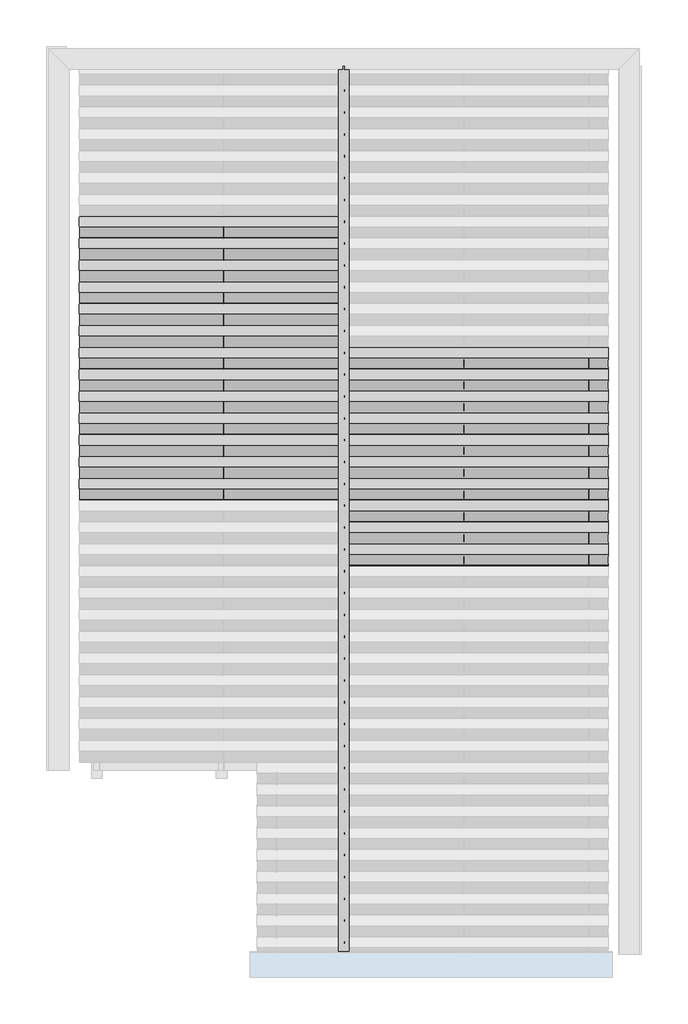
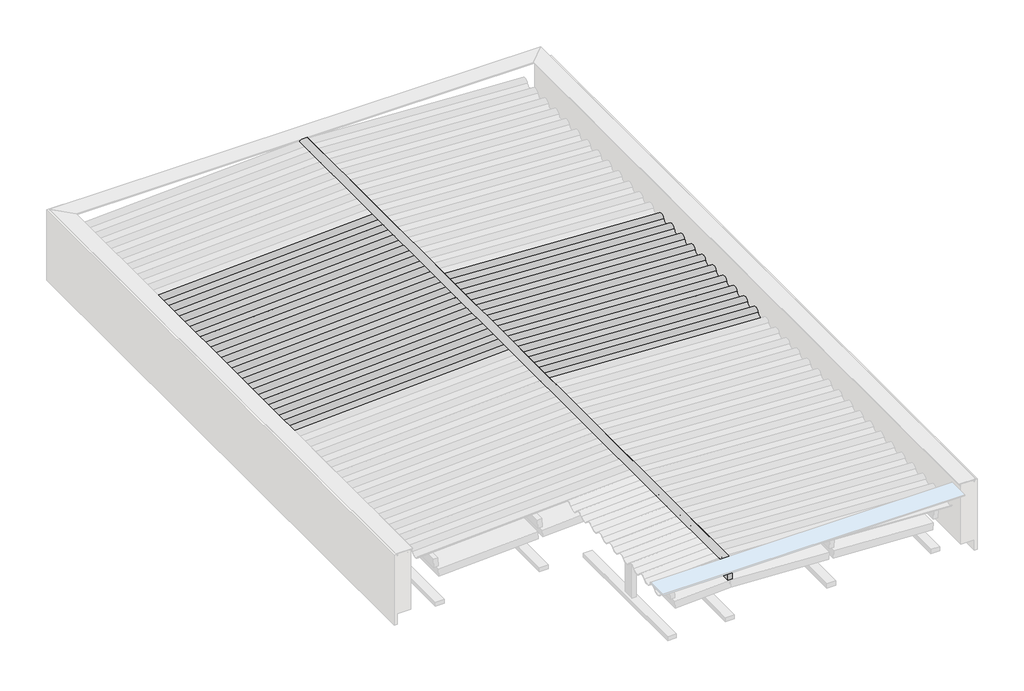
# One storey, part 3 of 4: 32 beams, 6 columns.
"""IFC4 building model written with IfcOpenShell, lengths in millimetres."""

import ifcopenshell
import ifcopenshell.guid

model = None  # the IFC model being written
_history = None  # IfcOwnerHistory: only IFC2X3 demands one
_inside = {}  # id of a spatial element -> (the spatial element, [elements in it])
_under = {}  # id of a project, library or spatial element -> (it, [spatial elements below it])
_declared = {}  # id of a project -> (the project, [libraries it declares])
_typed = {}  # id of a type object -> (the type object, [elements of that type])
_made_of = {}  # id of a material, layer set ... -> (it, [elements and type objects made of it])


def new_model(schema):
    """Start an empty IFC model of exactly this schema.

    Asked for "IFC4X3", IfcOpenShell would pick the latest addendum, in which some entities
    have other attributes; the version numbers below select the first issue.
    IFC2X3 requires an IfcOwnerHistory on every rooted entity: one is made here for all.
    """
    global model, _history
    if schema == "IFC4X3":
        model = ifcopenshell.file(schema_version=(4, 3, 0, 0))
    else:
        model = ifcopenshell.file(schema=schema)
    _inside.clear()
    _under.clear()
    _declared.clear()
    _typed.clear()
    _made_of.clear()
    _history = None
    if model.schema == "IFC2X3":
        org = make("IfcOrganization", Name="unknown")
        user = make(
            "IfcPersonAndOrganization",
            ThePerson=make("IfcPerson", FamilyName="unknown"),
            TheOrganization=org,
        )
        app = make(
            "IfcApplication",
            ApplicationDeveloper=org,
            Version="unknown",
            ApplicationFullName="unknown",
            ApplicationIdentifier="unknown",
        )
        _history = make(
            "IfcOwnerHistory",
            OwningUser=user,
            OwningApplication=app,
            ChangeAction="ADDED",
            CreationDate=0,
        )
    return model


def make(cls, **values):
    """One entity of the class cls with the attributes given. An attribute that is None is left unset."""
    return model.create_entity(
        cls, **{name: value for name, value in values.items() if value is not None}
    )


def rooted(cls, **values):
    """An entity with a GlobalId (a new one), such as an element, a storey or a relation."""
    return make(cls, GlobalId=ifcopenshell.guid.new(), OwnerHistory=_history, **values)


def si_unit(unit_type, name, prefix=None):
    """IfcSIUnit, for example si_unit("LENGTHUNIT", "METRE", prefix="MILLI")."""
    return make("IfcSIUnit", UnitType=unit_type, Prefix=prefix, Name=name)


def assignment(units):
    """IfcUnitAssignment: the units of a project."""
    return None if units is None else make("IfcUnitAssignment", Units=units)


def point(xyz):
    """IfcCartesianPoint."""
    return None if xyz is None else make("IfcCartesianPoint", Coordinates=xyz)


def direction(xyz):
    """IfcDirection."""
    return None if xyz is None else make("IfcDirection", DirectionRatios=xyz)


def frame(location, z_axis=None, x_axis=None):
    """IfcAxis2Placement3D, a coordinate frame: its origin and axes. An axis left out is left unset."""
    return make(
        "IfcAxis2Placement3D",
        Location=point(location),
        Axis=direction(z_axis),
        RefDirection=direction(x_axis),
    )


def frame_2d(location, x_axis=None):
    """IfcAxis2Placement2D, a coordinate frame in the plane: its origin and x axis."""
    return make(
        "IfcAxis2Placement2D", Location=point(location), RefDirection=direction(x_axis)
    )


def origin():
    """The frame at (0, 0, 0) with its axes left unset."""
    return frame((0.0, 0.0, 0.0))


def place(relative_to, where):
    """IfcLocalPlacement: puts the frame where relative to a parent placement (None: the world)."""
    return make(
        "IfcLocalPlacement", PlacementRelTo=relative_to, RelativePlacement=where
    )


def context(
    kind, dimensions, precision=None, world=None, true_north=None, identifier=None
):
    """IfcGeometricRepresentationContext, for example the 3D "Model" context."""
    return make(
        "IfcGeometricRepresentationContext",
        ContextIdentifier=identifier,
        ContextType=kind,
        CoordinateSpaceDimension=dimensions,
        Precision=precision,
        WorldCoordinateSystem=world,
        TrueNorth=true_north,
    )


def project(units=None, contexts=None):
    """IfcProject with its units and contexts."""
    return rooted(
        "IfcProject",
        Name="project",
        RepresentationContexts=contexts,
        UnitsInContext=assignment(units),
    )


def spatial(cls, under=None, at=None, **own):
    """A site, building, storey or space (cls), placed at a placement, below another one or the project."""
    s = rooted(cls, ObjectPlacement=at, **own)
    if under is not None:
        _under.setdefault(under.id(), (under, []))[1].append(s)
    return s


def polyline(points):
    """IfcPolyline through the points."""
    return make("IfcPolyline", Points=[point(p) for p in points])


def circle_curve(where, radius):
    """IfcCircle in the frame where."""
    return make("IfcCircle", Position=where, Radius=radius)


def trimmed(basis, trim1, trim2, sense, master):
    """IfcTrimmedCurve: the piece of a basis curve between two trims."""
    return make(
        "IfcTrimmedCurve",
        BasisCurve=basis,
        Trim1=trim1,
        Trim2=trim2,
        SenseAgreement=sense,
        MasterRepresentation=master,
    )


def segment(curve, same_sense, transition):
    """IfcCompositeCurveSegment."""
    return make(
        "IfcCompositeCurveSegment",
        Transition=transition,
        SameSense=same_sense,
        ParentCurve=curve,
    )


def composite_curve(segments, self_intersect=None):
    """IfcCompositeCurve: segments joined end to end."""
    return make("IfcCompositeCurve", Segments=segments, SelfIntersect=self_intersect)


def outline(outer, holes=None, kind="AREA"):
    """IfcArbitraryClosedProfileDef: a profile drawn as a closed curve; with holes, ...WithVoids."""
    if holes is None:
        return make("IfcArbitraryClosedProfileDef", ProfileType=kind, OuterCurve=outer)
    return make(
        "IfcArbitraryProfileDefWithVoids",
        ProfileType=kind,
        OuterCurve=outer,
        InnerCurves=holes,
    )


def extrude(swept, where, along, depth):
    """IfcExtrudedAreaSolid: the profile swept, set in the frame where, extruded along a direction by depth."""
    return make(
        "IfcExtrudedAreaSolid",
        SweptArea=swept,
        Position=where,
        ExtrudedDirection=direction(along),
        Depth=depth,
    )


def shape(context_of_items, identifier, shape_type, items):
    """IfcShapeRepresentation: the items that make up one representation, for example the "Body"."""
    return make(
        "IfcShapeRepresentation",
        ContextOfItems=context_of_items,
        RepresentationIdentifier=identifier,
        RepresentationType=shape_type,
        Items=items,
    )


def source(mapping_origin, context_of_items, identifier, shape_type, items):
    """IfcRepresentationMap: a shape defined once, which mapped items show again and again."""
    return make(
        "IfcRepresentationMap",
        MappingOrigin=mapping_origin,
        MappedRepresentation=shape(context_of_items, identifier, shape_type, items),
    )


def transform(
    local_origin,
    x_axis=None,
    y_axis=None,
    z_axis=None,
    scale=None,
    scale2=None,
    scale3=None,
    uniform=True,
):
    """IfcCartesianTransformationOperator3D, or its non-uniform kind. x_axis, y_axis, z_axis: its Axis1, 2, 3."""
    if uniform:
        return make(
            "IfcCartesianTransformationOperator3D",
            Axis1=direction(x_axis),
            Axis2=direction(y_axis),
            LocalOrigin=point(local_origin),
            Scale=scale,
            Axis3=direction(z_axis),
        )
    return make(
        "IfcCartesianTransformationOperator3DnonUniform",
        Axis1=direction(x_axis),
        Axis2=direction(y_axis),
        LocalOrigin=point(local_origin),
        Scale=scale,
        Axis3=direction(z_axis),
        Scale2=scale2,
        Scale3=scale3,
    )


def mapped(mapping_source, mapping_target):
    """IfcMappedItem: shows the shape of a source again, moved by a transform."""
    return make(
        "IfcMappedItem", MappingSource=mapping_source, MappingTarget=mapping_target
    )


def made_of(thing, what):
    """Note that an element or type object is made of a material, layer set ...; save() writes the relation."""
    if what is not None:
        _made_of.setdefault(what.id(), (what, []))[1].append(thing)
    return thing


def element(
    cls,
    number,
    at=None,
    inside=None,
    cuts=None,
    type_object=None,
    material=None,
    context=None,
    identifier="Body",
    shape_type=None,
    held_by="IfcProductDefinitionShape",
    body=None,
    shapes=None,
    **own,
):
    """One element of the class cls, such as IfcWall. Its Tag is "e" and its number.

    at: its placement. inside: the storey or other place that contains it. cuts: it is an
    opening in that element (IfcRelVoidsElement). A single representation is given by context,
    identifier, shape_type and body (its items); several are given by shapes. held_by: the class
    of the entity that holds the representations. save() writes the other relations.
    """
    e = rooted(cls, Tag="e%d" % number, ObjectPlacement=at, **own)
    if body is not None:
        shapes = [shape(context, identifier, shape_type, body)]
    if shapes is not None:
        e.Representation = make(held_by, Representations=shapes)
    if inside is not None:
        _inside.setdefault(inside.id(), (inside, []))[1].append(e)
    if cuts is not None:
        rooted(
            "IfcRelVoidsElement", RelatingBuildingElement=cuts, RelatedOpeningElement=e
        )
    if type_object is not None:
        _typed.setdefault(type_object.id(), (type_object, []))[1].append(e)
    return made_of(e, material)


def aggregate(whole, parts):
    """IfcRelAggregates: a whole, such as a stair, and the parts it consists of."""
    return rooted("IfcRelAggregates", RelatingObject=whole, RelatedObjects=parts)


def save(model, path):
    """Write the relations noted so far, then the file.

    IfcRelAggregates (storeys below a building ...), IfcRelContainedInSpatialStructure (elements
    in a storey), IfcRelDefinesByType, IfcRelAssociatesMaterial and IfcRelDeclares: one each for
    every whole, place, type object, material and project.
    """
    for whole, parts in _under.values():
        aggregate(whole, parts)
    for where, things in _inside.values():
        rooted(
            "IfcRelContainedInSpatialStructure",
            RelatedElements=things,
            RelatingStructure=where,
        )
    for kind, things in _typed.values():
        rooted("IfcRelDefinesByType", RelatedObjects=things, RelatingType=kind)
    for what, things in _made_of.values():
        rooted("IfcRelAssociatesMaterial", RelatedObjects=things, RelatingMaterial=what)
    for by, libraries in _declared.values():
        rooted("IfcRelDeclares", RelatingContext=by, RelatedDefinitions=libraries)
    model.write(path)


def cumeeira_telha_ondulada_fibrocimento_c9eafb3e(model_context):
    return source(origin(), model_context, "Body", "SweptSolid", [
        extrude(outline(composite_curve([segment(polyline([(58.3970135, 42.4437972), (53.9055884, 40.2467307)]), True, "CONTINUOUS"), segment(trimmed(circle_curve(frame_2d((-1.6029865, 13.0936483)), 61.7939461), [point((53.9055884, 40.2467307))], [point((-57.1115615, 40.2467307))], True, "CARTESIAN"), True, "CONTINUOUS"), segment(polyline([(-57.1115615, 40.2467307), (-61.6029865, 42.4437972)]), True, "CONTINUOUS"), segment(trimmed(circle_curve(frame_2d((-1.6029865, 13.0936483)), 66.7939461), [point((-61.6029865, 42.4437972))], [point((58.3970135, 42.4437972))], False, "CARTESIAN"), True, "CONTINUOUS")], self_intersect=False)), frame((-4969.5, 0.0, 0.0), z_axis=(1.0, 0.0, 0.0), x_axis=(0.0, 1.0, 0.0)), (0.0, 0.0, 1.0), 9939.0),
    ])


def viga_cumeeira_6x16cm_5eb8e513(model_context):
    return source(origin(), model_context, "Body", "SweptSolid", [
        extrude(outline(polyline([(4969.5, 30.0), (4969.5, -30.0), (-4969.5, -30.0), (-4969.5, 30.0), (4969.5, 30.0)])), frame((0.0, 0.0, -80.0), z_axis=(0.0, 0.0, 1.0), x_axis=(1.0, 0.0, 0.0)), (0.0, 0.0, 1.0), 160.0),
    ])


def column_f3930958(model_context):
    return source(origin(), model_context, "Body", "SweptSolid", [
        extrude(outline(polyline([(30.0, 80.0), (30.0, -80.0), (-30.0, -80.0), (-30.0, 80.0), (30.0, 80.0)])), frame((0.0, 0.0, 4460.0), z_axis=(0.0, 0.0, 1.0), x_axis=(1.0, 0.0, 0.0)), (0.0, 0.0, 1.0), 522.9),
    ])


def column_4d3918cc(model_context):
    return source(origin(), model_context, "Body", "SweptSolid", [
        extrude(outline(polyline([(30.0, 80.0), (30.0, -80.0), (-30.0, -80.0), (-30.0, 80.0), (30.0, 80.0)])), frame((0.0, 0.0, 4460.0), z_axis=(0.0, 0.0, 1.0), x_axis=(1.0, 0.0, 0.0)), (0.0, 0.0, 1.0), 426.9),
    ])


def column_924cc83b(model_context):
    return source(origin(), model_context, "Body", "SweptSolid", [
        extrude(outline(polyline([(30.0, 80.0), (30.0, -80.0), (-30.0, -80.0), (-30.0, 80.0), (30.0, 80.0)])), frame((0.0, 0.0, 4460.0), z_axis=(0.0, 0.0, 1.0), x_axis=(1.0, 0.0, 0.0)), (0.0, 0.0, 1.0), 497.0),
    ])


model = new_model("IFC4")

# Units and contexts
model_context = context("Model", 3, world=origin())
ifc_project = project(units=[si_unit("LENGTHUNIT", "METRE", prefix="MILLI")], contexts=[model_context])

# Site, building, storey
site = spatial("IfcSite", under=ifc_project)
building = spatial("IfcBuilding", under=site)
storey = spatial("IfcBuildingStorey", under=building, Name="COB. SALA ESTAR", Elevation=4400.0)

# Beams
placement = place(None, origin())
element("IfcBeam", 1, ObjectType="Madeira de lei : Berço 6x12cm", at=placement, inside=storey, context=model_context, shape_type="SweptSolid", body=[
    extrude(outline(polyline([(-3400.781307, 1623.9300153), (-3280.781307, 1623.9300153), (-3280.781307, -376.0699847), (-3400.781307, -376.0699847), (-3400.781307, 1623.9300153)])), frame((0.0, 0.0, 4400.0), z_axis=(0.0, 0.0, 1.0), x_axis=(1.0, 0.0, 0.0)), (0.0, 0.0, 1.0), 60.0),
])
element("IfcBeam", 2, ObjectType="Madeira de lei : Berço 6x12cm", at=placement, inside=storey, context=model_context, shape_type="SweptSolid", body=[
    extrude(outline(polyline([(-3400.781307, 3623.9300153), (-3280.781307, 3623.9300153), (-3280.781307, 1623.9300153), (-3400.781307, 1623.9300153), (-3400.781307, 3623.9300153)])), frame((0.0, 0.0, 4400.0), z_axis=(0.0, 0.0, 1.0), x_axis=(1.0, 0.0, 0.0)), (0.0, 0.0, 1.0), 60.0),
])
element("IfcBeam", 3, ObjectType="Madeira de lei : Berço 6x12cm", at=placement, inside=storey, context=model_context, shape_type="SweptSolid", body=[
    extrude(outline(polyline([(-2032.4438771, 1623.9300153), (-1912.4438771, 1623.9300153), (-1912.4438771, -376.0699847), (-2032.4438771, -376.0699847), (-2032.4438771, 1623.9300153)])), frame((0.0, 0.0, 4400.0), z_axis=(0.0, 0.0, 1.0), x_axis=(1.0, 0.0, 0.0)), (0.0, 0.0, 1.0), 60.0),
])
element("IfcBeam", 4, ObjectType="Madeira de lei : Berço 6x12cm", at=placement, inside=storey, context=model_context, shape_type="SweptSolid", body=[
    extrude(outline(polyline([(-634.1438771, 1623.9300153), (-514.1438771, 1623.9300153), (-514.1438771, -376.0699847), (-634.1438771, -376.0699847), (-634.1438771, 1623.9300153)])), frame((0.0, 0.0, 4400.0), z_axis=(0.0, 0.0, 1.0), x_axis=(1.0, 0.0, 0.0)), (0.0, 0.0, 1.0), 60.0),
])
element("IfcBeam", 5, ObjectType="Madeira de lei : Berço 6x12cm", at=placement, inside=storey, context=model_context, shape_type="SweptSolid", body=[
    extrude(outline(polyline([(-4769.1187368, 1623.9300153), (-4649.1187368, 1623.9300153), (-4649.1187368, -376.0699847), (-4769.1187368, -376.0699847), (-4769.1187368, 1623.9300153)])), frame((0.0, 0.0, 4400.0), z_axis=(0.0, 0.0, 1.0), x_axis=(1.0, 0.0, 0.0)), (0.0, 0.0, 1.0), 60.0),
])
element("IfcBeam", 6, ObjectType="Madeira de lei : Berço 6x12cm", at=placement, inside=storey, context=model_context, shape_type="SweptSolid", body=[
    extrude(outline(polyline([(-4769.1187368, 3623.9300153), (-4649.1187368, 3623.9300153), (-4649.1187368, 1623.9300153), (-4769.1187368, 1623.9300153), (-4769.1187368, 3623.9300153)])), frame((0.0, 0.0, 4400.0), z_axis=(0.0, 0.0, 1.0), x_axis=(1.0, 0.0, 0.0)), (0.0, 0.0, 1.0), 60.0),
])
element("IfcBeam", 7, ObjectType="Madeira de lei : Berço 6x12cm", at=placement, inside=storey, context=model_context, shape_type="SweptSolid", body=[
    extrude(outline(polyline([(-6167.4187368, 3623.9300153), (-6047.4187368, 3623.9300153), (-6047.4187368, 1623.9300153), (-6167.4187368, 1623.9300153), (-6167.4187368, 3623.9300153)])), frame((0.0, 0.0, 4400.0), z_axis=(0.0, 0.0, 1.0), x_axis=(1.0, 0.0, 0.0)), (0.0, 0.0, 1.0), 60.0),
])
cumeeira_telha_ondulada_fibrocimento_shape = cumeeira_telha_ondulada_fibrocimento_c9eafb3e(model_context)
element("IfcBeam", 8, ObjectType="Cumeeira Telha Ondulada : Fibrocimento", at=placement, inside=storey, context=model_context, shape_type="MappedRepresentation", body=[
    mapped(cumeeira_telha_ondulada_fibrocimento_shape, transform((-3340.781307, 623.9300153, 5182.0251229), x_axis=(0.0, -1.0, 0.0), y_axis=(1.0, 0.0, 0.0), z_axis=(0.0, 0.0, 1.0))),
])
element("IfcBeam", 9, ObjectType="Telha Ondulada : Fibrocimento", at=placement, inside=storey, context=model_context, shape_type="SweptSolid", body=[
    extrude(outline(composite_curve([segment(trimmed(circle_curve(frame_2d((-58.7002978, -53.2060538)), 66.7939461), [point((-29.3501488, 6.7939462))], [point((-29.3501488, -113.2060538))], False, "CARTESIAN"), True, "CONTINUOUS"), segment(polyline([(-29.3501488, -113.2060538), (-31.5472154, -108.7146288)]), True, "CONTINUOUS"), segment(trimmed(circle_curve(frame_2d((-58.7002978, -53.2060538)), 61.7939461), [point((-31.5472154, -108.7146288))], [point((-31.5472154, 2.3025211))], True, "CARTESIAN"), True, "CONTINUOUS"), segment(trimmed(circle_curve(frame_2d((0.0, 66.7939462)), 71.7939461), [point((-31.5472154, 2.3025211))], [point((-31.5472154, 131.2853712))], False, "CARTESIAN"), True, "CONTINUOUS"), segment(polyline([(-31.5472154, 131.2853712), (-29.3501488, 126.7939462)]), True, "CONTINUOUS"), segment(trimmed(circle_curve(frame_2d((0.0, 66.7939462)), 66.7939461), [point((-29.3501488, 126.7939462))], [point((-29.3501488, 6.7939462))], True, "CARTESIAN"), True, "CONTINUOUS")], self_intersect=False)), frame((-6303.6781287, 866.826948, 5068.1236978), z_axis=(0.9987523388778448, 0.0, 0.04993761694389134), x_axis=(-0.04993761694389134, 0.0, 0.9987523388778448)), (0.0, 0.0, 1.0), 2962.0084336),
])
element("IfcBeam", 10, ObjectType="Telha Ondulada : Fibrocimento", at=placement, inside=storey, context=model_context, shape_type="SweptSolid", body=[
    extrude(outline(composite_curve([segment(trimmed(circle_curve(frame_2d((-58.7002978, -53.2060538)), 66.7939461), [point((-29.3501488, 6.7939462))], [point((-29.3501488, -113.2060538))], False, "CARTESIAN"), True, "CONTINUOUS"), segment(polyline([(-29.3501488, -113.2060538), (-31.5472154, -108.7146288)]), True, "CONTINUOUS"), segment(trimmed(circle_curve(frame_2d((-58.7002978, -53.2060538)), 61.7939461), [point((-31.5472154, -108.7146288))], [point((-31.5472154, 2.3025211))], True, "CARTESIAN"), True, "CONTINUOUS"), segment(trimmed(circle_curve(frame_2d((0.0, 66.7939462)), 71.7939461), [point((-31.5472154, 2.3025211))], [point((-31.5472154, 131.2853712))], False, "CARTESIAN"), True, "CONTINUOUS"), segment(polyline([(-31.5472154, 131.2853712), (-29.3501488, 126.7939462)]), True, "CONTINUOUS"), segment(trimmed(circle_curve(frame_2d((0.0, 66.7939462)), 66.7939461), [point((-29.3501488, 126.7939462))], [point((-29.3501488, 6.7939462))], True, "CARTESIAN"), True, "CONTINUOUS")], self_intersect=False)), frame((-6303.6781287, 1111.326948, 5068.1236978), z_axis=(0.9987523388778448, 0.0, 0.04993761694389136), x_axis=(-0.04993761694389136, 0.0, 0.9987523388778448)), (0.0, 0.0, 1.0), 2962.0084336),
])
element("IfcBeam", 11, ObjectType="Telha Ondulada : Fibrocimento", at=placement, inside=storey, context=model_context, shape_type="SweptSolid", body=[
    extrude(outline(composite_curve([segment(trimmed(circle_curve(frame_2d((-58.7002978, -53.2060538)), 66.7939461), [point((-29.3501488, 6.7939462))], [point((-29.3501488, -113.2060538))], False, "CARTESIAN"), True, "CONTINUOUS"), segment(polyline([(-29.3501488, -113.2060538), (-31.5472154, -108.7146288)]), True, "CONTINUOUS"), segment(trimmed(circle_curve(frame_2d((-58.7002978, -53.2060538)), 61.7939461), [point((-31.5472154, -108.7146288))], [point((-31.5472154, 2.3025211))], True, "CARTESIAN"), True, "CONTINUOUS"), segment(trimmed(circle_curve(frame_2d((0.0, 66.7939462)), 71.7939461), [point((-31.5472154, 2.3025211))], [point((-31.5472154, 131.2853712))], False, "CARTESIAN"), True, "CONTINUOUS"), segment(polyline([(-31.5472154, 131.2853712), (-29.3501488, 126.7939462)]), True, "CONTINUOUS"), segment(trimmed(circle_curve(frame_2d((0.0, 66.7939462)), 66.7939461), [point((-29.3501488, 126.7939462))], [point((-29.3501488, 6.7939462))], True, "CARTESIAN"), True, "CONTINUOUS")], self_intersect=False)), frame((-6303.6781287, 1355.826948, 5068.1236978), z_axis=(0.9987523388778448, 0.0, 0.04993761694389134), x_axis=(-0.04993761694389134, 0.0, 0.9987523388778448)), (0.0, 0.0, 1.0), 2962.0084336),
])
element("IfcBeam", 12, ObjectType="Telha Ondulada : Fibrocimento", at=placement, inside=storey, context=model_context, shape_type="SweptSolid", body=[
    extrude(outline(composite_curve([segment(trimmed(circle_curve(frame_2d((-58.7002978, -53.2060538)), 66.7939461), [point((-29.3501488, 6.7939462))], [point((-29.3501488, -113.2060538))], False, "CARTESIAN"), True, "CONTINUOUS"), segment(polyline([(-29.3501488, -113.2060538), (-31.5472154, -108.7146288)]), True, "CONTINUOUS"), segment(trimmed(circle_curve(frame_2d((-58.7002978, -53.2060538)), 61.7939461), [point((-31.5472154, -108.7146288))], [point((-31.5472154, 2.3025211))], True, "CARTESIAN"), True, "CONTINUOUS"), segment(trimmed(circle_curve(frame_2d((0.0, 66.7939462)), 71.7939461), [point((-31.5472154, 2.3025211))], [point((-31.5472154, 131.2853712))], False, "CARTESIAN"), True, "CONTINUOUS"), segment(polyline([(-31.5472154, 131.2853712), (-29.3501488, 126.7939462)]), True, "CONTINUOUS"), segment(trimmed(circle_curve(frame_2d((0.0, 66.7939462)), 66.7939461), [point((-29.3501488, 126.7939462))], [point((-29.3501488, 6.7939462))], True, "CARTESIAN"), True, "CONTINUOUS")], self_intersect=False)), frame((-6303.6781287, 1600.326948, 5068.1236978), z_axis=(0.9987523388778448, 0.0, 0.04993761694389136), x_axis=(-0.04993761694389136, 0.0, 0.9987523388778448)), (0.0, 0.0, 1.0), 2962.0084336),
])
element("IfcBeam", 13, ObjectType="Telha Ondulada : Fibrocimento", at=placement, inside=storey, context=model_context, shape_type="SweptSolid", body=[
    extrude(outline(composite_curve([segment(trimmed(circle_curve(frame_2d((-58.7002978, -53.2060538)), 66.7939461), [point((-29.3501488, 6.7939462))], [point((-29.3501488, -113.2060538))], False, "CARTESIAN"), True, "CONTINUOUS"), segment(polyline([(-29.3501488, -113.2060538), (-31.5472154, -108.7146288)]), True, "CONTINUOUS"), segment(trimmed(circle_curve(frame_2d((-58.7002978, -53.2060538)), 61.7939461), [point((-31.5472154, -108.7146288))], [point((-31.5472154, 2.3025211))], True, "CARTESIAN"), True, "CONTINUOUS"), segment(trimmed(circle_curve(frame_2d((0.0, 66.7939462)), 71.7939461), [point((-31.5472154, 2.3025211))], [point((-31.5472154, 131.2853712))], False, "CARTESIAN"), True, "CONTINUOUS"), segment(polyline([(-31.5472154, 131.2853712), (-29.3501488, 126.7939462)]), True, "CONTINUOUS"), segment(trimmed(circle_curve(frame_2d((0.0, 66.7939462)), 66.7939461), [point((-29.3501488, 126.7939462))], [point((-29.3501488, 6.7939462))], True, "CARTESIAN"), True, "CONTINUOUS")], self_intersect=False)), frame((-6303.6781287, 1844.826948, 5068.1236978), z_axis=(0.9987523388778448, 0.0, 0.049937616943891344), x_axis=(-0.049937616943891344, 0.0, 0.9987523388778448)), (0.0, 0.0, 1.0), 2962.0084336),
])
element("IfcBeam", 14, ObjectType="Telha Ondulada : Fibrocimento", at=placement, inside=storey, context=model_context, shape_type="SweptSolid", body=[
    extrude(outline(composite_curve([segment(trimmed(circle_curve(frame_2d((-58.7002978, -53.2060538)), 66.7939461), [point((-29.3501488, 6.7939462))], [point((-29.3501488, -113.2060538))], False, "CARTESIAN"), True, "CONTINUOUS"), segment(polyline([(-29.3501488, -113.2060538), (-31.5472154, -108.7146288)]), True, "CONTINUOUS"), segment(trimmed(circle_curve(frame_2d((-58.7002978, -53.2060538)), 61.7939461), [point((-31.5472154, -108.7146288))], [point((-31.5472154, 2.3025211))], True, "CARTESIAN"), True, "CONTINUOUS"), segment(trimmed(circle_curve(frame_2d((0.0, 66.7939462)), 71.7939461), [point((-31.5472154, 2.3025211))], [point((-31.5472154, 131.2853712))], False, "CARTESIAN"), True, "CONTINUOUS"), segment(polyline([(-31.5472154, 131.2853712), (-29.3501488, 126.7939462)]), True, "CONTINUOUS"), segment(trimmed(circle_curve(frame_2d((0.0, 66.7939462)), 66.7939461), [point((-29.3501488, 126.7939462))], [point((-29.3501488, 6.7939462))], True, "CARTESIAN"), True, "CONTINUOUS")], self_intersect=False)), frame((-6303.6781287, 2089.326948, 5068.1236978), z_axis=(0.9987523388778448, 0.0, 0.04993761694389134), x_axis=(-0.04993761694389134, 0.0, 0.9987523388778448)), (0.0, 0.0, 1.0), 2962.0084336),
])
element("IfcBeam", 15, ObjectType="Telha Ondulada : Fibrocimento", at=placement, inside=storey, context=model_context, shape_type="SweptSolid", body=[
    extrude(outline(composite_curve([segment(trimmed(circle_curve(frame_2d((-58.7002978, -53.2060538)), 66.7939461), [point((-29.3501488, 6.7939462))], [point((-29.3501488, -113.2060538))], False, "CARTESIAN"), True, "CONTINUOUS"), segment(polyline([(-29.3501488, -113.2060538), (-31.5472154, -108.7146288)]), True, "CONTINUOUS"), segment(trimmed(circle_curve(frame_2d((-58.7002978, -53.2060538)), 61.7939461), [point((-31.5472154, -108.7146288))], [point((-31.5472154, 2.3025211))], True, "CARTESIAN"), True, "CONTINUOUS"), segment(trimmed(circle_curve(frame_2d((0.0, 66.7939462)), 71.7939461), [point((-31.5472154, 2.3025211))], [point((-31.5472154, 131.2853712))], False, "CARTESIAN"), True, "CONTINUOUS"), segment(polyline([(-31.5472154, 131.2853712), (-29.3501488, 126.7939462)]), True, "CONTINUOUS"), segment(trimmed(circle_curve(frame_2d((0.0, 66.7939462)), 66.7939461), [point((-29.3501488, 126.7939462))], [point((-29.3501488, 6.7939462))], True, "CARTESIAN"), True, "CONTINUOUS")], self_intersect=False)), frame((-6303.6781287, 2333.826948, 5068.1236978), z_axis=(0.9987523388778448, 0.0, 0.04993761694389136), x_axis=(-0.04993761694389136, 0.0, 0.9987523388778448)), (0.0, 0.0, 1.0), 2962.0084336),
])
element("IfcBeam", 16, ObjectType="Telha Ondulada : Fibrocimento", at=placement, inside=storey, context=model_context, shape_type="SweptSolid", body=[
    extrude(outline(composite_curve([segment(trimmed(circle_curve(frame_2d((-58.7002978, -53.2060538)), 66.7939461), [point((-29.3501488, 6.7939462))], [point((-29.3501488, -113.2060538))], False, "CARTESIAN"), True, "CONTINUOUS"), segment(polyline([(-29.3501488, -113.2060538), (-31.5472154, -108.7146288)]), True, "CONTINUOUS"), segment(trimmed(circle_curve(frame_2d((-58.7002978, -53.2060538)), 61.7939461), [point((-31.5472154, -108.7146288))], [point((-31.5472154, 2.3025211))], True, "CARTESIAN"), True, "CONTINUOUS"), segment(trimmed(circle_curve(frame_2d((0.0, 66.7939462)), 71.7939461), [point((-31.5472154, 2.3025211))], [point((-31.5472154, 131.2853712))], False, "CARTESIAN"), True, "CONTINUOUS"), segment(polyline([(-31.5472154, 131.2853712), (-29.3501488, 126.7939462)]), True, "CONTINUOUS"), segment(trimmed(circle_curve(frame_2d((0.0, 66.7939462)), 66.7939461), [point((-29.3501488, 126.7939462))], [point((-29.3501488, 6.7939462))], True, "CARTESIAN"), True, "CONTINUOUS")], self_intersect=False)), frame((-6303.6781287, 2578.326948, 5068.1236978), z_axis=(0.9987523388778448, 0.0, 0.04993761694389134), x_axis=(-0.04993761694389134, 0.0, 0.9987523388778448)), (0.0, 0.0, 1.0), 2962.0084336),
])
element("IfcBeam", 17, ObjectType="Telha Ondulada : Fibrocimento", at=placement, inside=storey, context=model_context, shape_type="SweptSolid", body=[
    extrude(outline(composite_curve([segment(trimmed(circle_curve(frame_2d((-58.7002978, -53.2060538)), 66.7939461), [point((-29.3501488, 6.7939462))], [point((-29.3501488, -113.2060538))], False, "CARTESIAN"), True, "CONTINUOUS"), segment(polyline([(-29.3501488, -113.2060538), (-31.5472154, -108.7146288)]), True, "CONTINUOUS"), segment(trimmed(circle_curve(frame_2d((-58.7002978, -53.2060538)), 61.7939461), [point((-31.5472154, -108.7146288))], [point((-31.5472154, 2.3025211))], True, "CARTESIAN"), True, "CONTINUOUS"), segment(trimmed(circle_curve(frame_2d((0.0, 66.7939462)), 71.7939461), [point((-31.5472154, 2.3025211))], [point((-31.5472154, 131.2853712))], False, "CARTESIAN"), True, "CONTINUOUS"), segment(polyline([(-31.5472154, 131.2853712), (-29.3501488, 126.7939462)]), True, "CONTINUOUS"), segment(trimmed(circle_curve(frame_2d((0.0, 66.7939462)), 66.7939461), [point((-29.3501488, 126.7939462))], [point((-29.3501488, 6.7939462))], True, "CARTESIAN"), True, "CONTINUOUS")], self_intersect=False)), frame((-6303.6781287, 2822.826948, 5068.1236978), z_axis=(0.9987523388778448, 0.0, 0.04993761694389136), x_axis=(-0.04993761694389136, 0.0, 0.9987523388778448)), (0.0, 0.0, 1.0), 2962.0084336),
])
element("IfcBeam", 18, ObjectType="Telha Ondulada : Fibrocimento", at=placement, inside=storey, context=model_context, shape_type="SweptSolid", body=[
    extrude(outline(composite_curve([segment(trimmed(circle_curve(frame_2d((-58.7002978, -53.2060538)), 66.7939461), [point((-29.3501488, 6.7939462))], [point((-29.3501488, -113.2060538))], False, "CARTESIAN"), True, "CONTINUOUS"), segment(polyline([(-29.3501488, -113.2060538), (-31.5472154, -108.7146288)]), True, "CONTINUOUS"), segment(trimmed(circle_curve(frame_2d((-58.7002978, -53.2060538)), 61.7939461), [point((-31.5472154, -108.7146288))], [point((-31.5472154, 2.3025211))], True, "CARTESIAN"), True, "CONTINUOUS"), segment(trimmed(circle_curve(frame_2d((0.0, 66.7939462)), 71.7939461), [point((-31.5472154, 2.3025211))], [point((-31.5472154, 131.2853712))], False, "CARTESIAN"), True, "CONTINUOUS"), segment(polyline([(-31.5472154, 131.2853712), (-29.3501488, 126.7939462)]), True, "CONTINUOUS"), segment(trimmed(circle_curve(frame_2d((0.0, 66.7939462)), 66.7939461), [point((-29.3501488, 126.7939462))], [point((-29.3501488, 6.7939462))], True, "CARTESIAN"), True, "CONTINUOUS")], self_intersect=False)), frame((-6303.6781287, 3067.326948, 5068.1236978), z_axis=(0.9987523388778448, 0.0, 0.04993761694389134), x_axis=(-0.04993761694389134, 0.0, 0.9987523388778448)), (0.0, 0.0, 1.0), 2962.0084336),
])
element("IfcBeam", 19, ObjectType="Telha Ondulada : Fibrocimento", at=placement, inside=storey, context=model_context, shape_type="SweptSolid", body=[
    extrude(outline(composite_curve([segment(trimmed(circle_curve(frame_2d((-58.7002978, -53.2060538)), 66.7939461), [point((-29.3501488, 6.7939462))], [point((-29.3501488, -113.2060538))], False, "CARTESIAN"), True, "CONTINUOUS"), segment(polyline([(-29.3501488, -113.2060538), (-31.5472154, -108.7146288)]), True, "CONTINUOUS"), segment(trimmed(circle_curve(frame_2d((-58.7002978, -53.2060538)), 61.7939461), [point((-31.5472154, -108.7146288))], [point((-31.5472154, 2.3025211))], True, "CARTESIAN"), True, "CONTINUOUS"), segment(trimmed(circle_curve(frame_2d((0.0, 66.7939462)), 71.7939461), [point((-31.5472154, 2.3025211))], [point((-31.5472154, 131.2853712))], False, "CARTESIAN"), True, "CONTINUOUS"), segment(polyline([(-31.5472154, 131.2853712), (-29.3501488, 126.7939462)]), True, "CONTINUOUS"), segment(trimmed(circle_curve(frame_2d((0.0, 66.7939462)), 66.7939461), [point((-29.3501488, 126.7939462))], [point((-29.3501488, 6.7939462))], True, "CARTESIAN"), True, "CONTINUOUS")], self_intersect=False)), frame((-6303.6781287, 3311.826948, 5068.1236978), z_axis=(0.9987523388778448, 0.0, 0.04993761694389133), x_axis=(-0.04993761694389133, 0.0, 0.9987523388778448)), (0.0, 0.0, 1.0), 2962.0084336),
])
element("IfcBeam", 20, ObjectType="Telha Ondulada : Fibrocimento", at=placement, inside=storey, context=model_context, shape_type="SweptSolid", body=[
    extrude(outline(composite_curve([segment(trimmed(circle_curve(frame_2d((-58.7002978, -53.2060538)), 66.7939461), [point((-29.3501488, 6.7939462))], [point((-29.3501488, -113.2060538))], False, "CARTESIAN"), True, "CONTINUOUS"), segment(polyline([(-29.3501488, -113.2060538), (-31.5472154, -108.7146288)]), True, "CONTINUOUS"), segment(trimmed(circle_curve(frame_2d((-58.7002978, -53.2060538)), 61.7939461), [point((-31.5472154, -108.7146288))], [point((-31.5472154, 2.3025211))], True, "CARTESIAN"), True, "CONTINUOUS"), segment(trimmed(circle_curve(frame_2d((0.0, 66.7939462)), 71.7939461), [point((-31.5472154, 2.3025211))], [point((-31.5472154, 131.2853712))], False, "CARTESIAN"), True, "CONTINUOUS"), segment(polyline([(-31.5472154, 131.2853712), (-29.3501488, 126.7939462)]), True, "CONTINUOUS"), segment(trimmed(circle_curve(frame_2d((0.0, 66.7939462)), 66.7939461), [point((-29.3501488, 126.7939462))], [point((-29.3501488, 6.7939462))], True, "CARTESIAN"), True, "CONTINUOUS")], self_intersect=False)), frame((-6303.6781287, 3556.326948, 5068.1236978), z_axis=(0.9987523388778448, 0.0, 0.049937616943891344), x_axis=(-0.049937616943891344, 0.0, 0.9987523388778448)), (0.0, 0.0, 1.0), 2962.0084336),
])
element("IfcBeam", 21, ObjectType="Telha Ondulada : Fibrocimento", at=placement, inside=storey, context=model_context, shape_type="SweptSolid", body=[
    extrude(outline(composite_curve([segment(trimmed(circle_curve(frame_2d((-58.7002978, -53.2060538)), 66.7939461), [point((-29.3501488, 6.7939462))], [point((-29.3501488, -113.2060538))], False, "CARTESIAN"), True, "CONTINUOUS"), segment(polyline([(-29.3501488, -113.2060538), (-31.5472154, -108.7146288)]), True, "CONTINUOUS"), segment(trimmed(circle_curve(frame_2d((-58.7002978, -53.2060538)), 61.7939461), [point((-31.5472154, -108.7146288))], [point((-31.5472154, 2.3025211))], True, "CARTESIAN"), True, "CONTINUOUS"), segment(trimmed(circle_curve(frame_2d((0.0, 66.7939462)), 71.7939461), [point((-31.5472154, 2.3025211))], [point((-31.5472154, 131.2853712))], False, "CARTESIAN"), True, "CONTINUOUS"), segment(polyline([(-31.5472154, 131.2853712), (-29.3501488, 126.7939462)]), True, "CONTINUOUS"), segment(trimmed(circle_curve(frame_2d((0.0, 66.7939462)), 66.7939461), [point((-29.3501488, 126.7939462))], [point((-29.3501488, 6.7939462))], True, "CARTESIAN"), True, "CONTINUOUS")], self_intersect=False)), frame((-6303.6781287, 3800.826948, 5068.1236978), z_axis=(0.9987523388778448, 0.0, 0.04993761694389134), x_axis=(-0.04993761694389134, 0.0, 0.9987523388778448)), (0.0, 0.0, 1.0), 2962.0084336),
])
element("IfcBeam", 22, ObjectType="Telha Ondulada : Fibrocimento", at=placement, inside=storey, context=model_context, shape_type="SweptSolid", body=[
    extrude(outline(composite_curve([segment(trimmed(circle_curve(frame_2d((0.0, 66.7939462)), 66.7939461), [point((29.3501488, 6.7939462))], [point((29.3501488, 126.7939462))], True, "CARTESIAN"), True, "CONTINUOUS"), segment(polyline([(29.3501488, 126.7939462), (31.5472154, 131.2853712)]), True, "CONTINUOUS"), segment(trimmed(circle_curve(frame_2d((0.0, 66.7939462)), 71.7939461), [point((31.5472154, 131.2853712))], [point((31.5472154, 2.3025211))], False, "CARTESIAN"), True, "CONTINUOUS"), segment(trimmed(circle_curve(frame_2d((58.7002978, -53.2060538)), 61.7939461), [point((31.5472154, 2.3025211))], [point((31.5472154, -108.7146288))], True, "CARTESIAN"), True, "CONTINUOUS"), segment(polyline([(31.5472154, -108.7146288), (29.3501488, -113.2060538)]), True, "CONTINUOUS"), segment(trimmed(circle_curve(frame_2d((58.7002978, -53.2060538)), 66.7939461), [point((29.3501488, -113.2060538))], [point((29.3501488, 6.7939462))], False, "CARTESIAN"), True, "CONTINUOUS")], self_intersect=False)), frame((-377.8844852, 133.326948, 5068.1236978), z_axis=(-0.9987523388778448, 0.0, 0.04993761694389145), x_axis=(-0.04993761694389145, 0.0, -0.9987523388778448)), (0.0, 0.0, 1.0), 2962.0084336),
])
element("IfcBeam", 23, ObjectType="Telha Ondulada : Fibrocimento", at=placement, inside=storey, context=model_context, shape_type="SweptSolid", body=[
    extrude(outline(composite_curve([segment(trimmed(circle_curve(frame_2d((0.0, 66.7939462)), 66.7939461), [point((29.3501488, 6.7939462))], [point((29.3501488, 126.7939462))], True, "CARTESIAN"), True, "CONTINUOUS"), segment(polyline([(29.3501488, 126.7939462), (31.5472154, 131.2853712)]), True, "CONTINUOUS"), segment(trimmed(circle_curve(frame_2d((0.0, 66.7939462)), 71.7939461), [point((31.5472154, 131.2853712))], [point((31.5472154, 2.3025211))], False, "CARTESIAN"), True, "CONTINUOUS"), segment(trimmed(circle_curve(frame_2d((58.7002978, -53.2060538)), 61.7939461), [point((31.5472154, 2.3025211))], [point((31.5472154, -108.7146288))], True, "CARTESIAN"), True, "CONTINUOUS"), segment(polyline([(31.5472154, -108.7146288), (29.3501488, -113.2060538)]), True, "CONTINUOUS"), segment(trimmed(circle_curve(frame_2d((58.7002978, -53.2060538)), 66.7939461), [point((29.3501488, -113.2060538))], [point((29.3501488, 6.7939462))], False, "CARTESIAN"), True, "CONTINUOUS")], self_intersect=False)), frame((-377.8844852, 377.826948, 5068.1236978), z_axis=(-0.9987523388778448, 0.0, 0.04993761694389145), x_axis=(-0.04993761694389145, 0.0, -0.9987523388778448)), (0.0, 0.0, 1.0), 2962.0084336),
])
element("IfcBeam", 24, ObjectType="Telha Ondulada : Fibrocimento", at=placement, inside=storey, context=model_context, shape_type="SweptSolid", body=[
    extrude(outline(composite_curve([segment(trimmed(circle_curve(frame_2d((0.0, 66.7939462)), 66.7939461), [point((29.3501488, 6.7939462))], [point((29.3501488, 126.7939462))], True, "CARTESIAN"), True, "CONTINUOUS"), segment(polyline([(29.3501488, 126.7939462), (31.5472154, 131.2853712)]), True, "CONTINUOUS"), segment(trimmed(circle_curve(frame_2d((0.0, 66.7939462)), 71.7939461), [point((31.5472154, 131.2853712))], [point((31.5472154, 2.3025211))], False, "CARTESIAN"), True, "CONTINUOUS"), segment(trimmed(circle_curve(frame_2d((58.7002978, -53.2060538)), 61.7939461), [point((31.5472154, 2.3025211))], [point((31.5472154, -108.7146288))], True, "CARTESIAN"), True, "CONTINUOUS"), segment(polyline([(31.5472154, -108.7146288), (29.3501488, -113.2060538)]), True, "CONTINUOUS"), segment(trimmed(circle_curve(frame_2d((58.7002978, -53.2060538)), 66.7939461), [point((29.3501488, -113.2060538))], [point((29.3501488, 6.7939462))], False, "CARTESIAN"), True, "CONTINUOUS")], self_intersect=False)), frame((-377.8844852, 622.326948, 5068.1236978), z_axis=(-0.9987523388778448, 0.0, 0.049937616943891455), x_axis=(-0.049937616943891455, 0.0, -0.9987523388778448)), (0.0, 0.0, 1.0), 2962.0084336),
])
element("IfcBeam", 25, ObjectType="Telha Ondulada : Fibrocimento", at=placement, inside=storey, context=model_context, shape_type="SweptSolid", body=[
    extrude(outline(composite_curve([segment(trimmed(circle_curve(frame_2d((0.0, 66.7939462)), 66.7939461), [point((29.3501488, 6.7939462))], [point((29.3501488, 126.7939462))], True, "CARTESIAN"), True, "CONTINUOUS"), segment(polyline([(29.3501488, 126.7939462), (31.5472154, 131.2853712)]), True, "CONTINUOUS"), segment(trimmed(circle_curve(frame_2d((0.0, 66.7939462)), 71.7939461), [point((31.5472154, 131.2853712))], [point((31.5472154, 2.3025211))], False, "CARTESIAN"), True, "CONTINUOUS"), segment(trimmed(circle_curve(frame_2d((58.7002978, -53.2060538)), 61.7939461), [point((31.5472154, 2.3025211))], [point((31.5472154, -108.7146288))], True, "CARTESIAN"), True, "CONTINUOUS"), segment(polyline([(31.5472154, -108.7146288), (29.3501488, -113.2060538)]), True, "CONTINUOUS"), segment(trimmed(circle_curve(frame_2d((58.7002978, -53.2060538)), 66.7939461), [point((29.3501488, -113.2060538))], [point((29.3501488, 6.7939462))], False, "CARTESIAN"), True, "CONTINUOUS")], self_intersect=False)), frame((-377.8844852, 866.826948, 5068.1236978), z_axis=(-0.9987523388778448, 0.0, 0.049937616943891455), x_axis=(-0.049937616943891455, 0.0, -0.9987523388778448)), (0.0, 0.0, 1.0), 2962.0084336),
])
element("IfcBeam", 26, ObjectType="Telha Ondulada : Fibrocimento", at=placement, inside=storey, context=model_context, shape_type="SweptSolid", body=[
    extrude(outline(composite_curve([segment(trimmed(circle_curve(frame_2d((0.0, 66.7939462)), 66.7939461), [point((29.3501488, 6.7939462))], [point((29.3501488, 126.7939462))], True, "CARTESIAN"), True, "CONTINUOUS"), segment(polyline([(29.3501488, 126.7939462), (31.5472154, 131.2853712)]), True, "CONTINUOUS"), segment(trimmed(circle_curve(frame_2d((0.0, 66.7939462)), 71.7939461), [point((31.5472154, 131.2853712))], [point((31.5472154, 2.3025211))], False, "CARTESIAN"), True, "CONTINUOUS"), segment(trimmed(circle_curve(frame_2d((58.7002978, -53.2060538)), 61.7939461), [point((31.5472154, 2.3025211))], [point((31.5472154, -108.7146288))], True, "CARTESIAN"), True, "CONTINUOUS"), segment(polyline([(31.5472154, -108.7146288), (29.3501488, -113.2060538)]), True, "CONTINUOUS"), segment(trimmed(circle_curve(frame_2d((58.7002978, -53.2060538)), 66.7939461), [point((29.3501488, -113.2060538))], [point((29.3501488, 6.7939462))], False, "CARTESIAN"), True, "CONTINUOUS")], self_intersect=False)), frame((-377.8844852, 1111.326948, 5068.1236978), z_axis=(-0.9987523388778448, 0.0, 0.049937616943891455), x_axis=(-0.049937616943891455, 0.0, -0.9987523388778448)), (0.0, 0.0, 1.0), 2962.0084336),
])
element("IfcBeam", 27, ObjectType="Telha Ondulada : Fibrocimento", at=placement, inside=storey, context=model_context, shape_type="SweptSolid", body=[
    extrude(outline(composite_curve([segment(trimmed(circle_curve(frame_2d((0.0, 66.7939462)), 66.7939461), [point((29.3501488, 6.7939462))], [point((29.3501488, 126.7939462))], True, "CARTESIAN"), True, "CONTINUOUS"), segment(polyline([(29.3501488, 126.7939462), (31.5472154, 131.2853712)]), True, "CONTINUOUS"), segment(trimmed(circle_curve(frame_2d((0.0, 66.7939462)), 71.7939461), [point((31.5472154, 131.2853712))], [point((31.5472154, 2.3025211))], False, "CARTESIAN"), True, "CONTINUOUS"), segment(trimmed(circle_curve(frame_2d((58.7002978, -53.2060538)), 61.7939461), [point((31.5472154, 2.3025211))], [point((31.5472154, -108.7146288))], True, "CARTESIAN"), True, "CONTINUOUS"), segment(polyline([(31.5472154, -108.7146288), (29.3501488, -113.2060538)]), True, "CONTINUOUS"), segment(trimmed(circle_curve(frame_2d((58.7002978, -53.2060538)), 66.7939461), [point((29.3501488, -113.2060538))], [point((29.3501488, 6.7939462))], False, "CARTESIAN"), True, "CONTINUOUS")], self_intersect=False)), frame((-377.8844852, 1355.826948, 5068.1236978), z_axis=(-0.9987523388778448, 0.0, 0.049937616943891455), x_axis=(-0.049937616943891455, 0.0, -0.9987523388778448)), (0.0, 0.0, 1.0), 2962.0084336),
])
element("IfcBeam", 28, ObjectType="Telha Ondulada : Fibrocimento", at=placement, inside=storey, context=model_context, shape_type="SweptSolid", body=[
    extrude(outline(composite_curve([segment(trimmed(circle_curve(frame_2d((0.0, 66.7939462)), 66.7939461), [point((29.3501488, 6.7939462))], [point((29.3501488, 126.7939462))], True, "CARTESIAN"), True, "CONTINUOUS"), segment(polyline([(29.3501488, 126.7939462), (31.5472154, 131.2853712)]), True, "CONTINUOUS"), segment(trimmed(circle_curve(frame_2d((0.0, 66.7939462)), 71.7939461), [point((31.5472154, 131.2853712))], [point((31.5472154, 2.3025211))], False, "CARTESIAN"), True, "CONTINUOUS"), segment(trimmed(circle_curve(frame_2d((58.7002978, -53.2060538)), 61.7939461), [point((31.5472154, 2.3025211))], [point((31.5472154, -108.7146288))], True, "CARTESIAN"), True, "CONTINUOUS"), segment(polyline([(31.5472154, -108.7146288), (29.3501488, -113.2060538)]), True, "CONTINUOUS"), segment(trimmed(circle_curve(frame_2d((58.7002978, -53.2060538)), 66.7939461), [point((29.3501488, -113.2060538))], [point((29.3501488, 6.7939462))], False, "CARTESIAN"), True, "CONTINUOUS")], self_intersect=False)), frame((-377.8844852, 1600.326948, 5068.1236978), z_axis=(-0.9987523388778448, 0.0, 0.049937616943891455), x_axis=(-0.049937616943891455, 0.0, -0.9987523388778448)), (0.0, 0.0, 1.0), 2962.0084336),
])
element("IfcBeam", 29, ObjectType="Telha Ondulada : Fibrocimento", at=placement, inside=storey, context=model_context, shape_type="SweptSolid", body=[
    extrude(outline(composite_curve([segment(trimmed(circle_curve(frame_2d((0.0, 66.7939462)), 66.7939461), [point((29.3501488, 6.7939462))], [point((29.3501488, 126.7939462))], True, "CARTESIAN"), True, "CONTINUOUS"), segment(polyline([(29.3501488, 126.7939462), (31.5472154, 131.2853712)]), True, "CONTINUOUS"), segment(trimmed(circle_curve(frame_2d((0.0, 66.7939462)), 71.7939461), [point((31.5472154, 131.2853712))], [point((31.5472154, 2.3025211))], False, "CARTESIAN"), True, "CONTINUOUS"), segment(trimmed(circle_curve(frame_2d((58.7002978, -53.2060538)), 61.7939461), [point((31.5472154, 2.3025211))], [point((31.5472154, -108.7146288))], True, "CARTESIAN"), True, "CONTINUOUS"), segment(polyline([(31.5472154, -108.7146288), (29.3501488, -113.2060538)]), True, "CONTINUOUS"), segment(trimmed(circle_curve(frame_2d((58.7002978, -53.2060538)), 66.7939461), [point((29.3501488, -113.2060538))], [point((29.3501488, 6.7939462))], False, "CARTESIAN"), True, "CONTINUOUS")], self_intersect=False)), frame((-377.8844852, 1844.826948, 5068.1236978), z_axis=(-0.9987523388778448, 0.0, 0.049937616943891455), x_axis=(-0.049937616943891455, 0.0, -0.9987523388778448)), (0.0, 0.0, 1.0), 2962.0084336),
])
element("IfcBeam", 30, ObjectType="Telha Ondulada : Fibrocimento", at=placement, inside=storey, context=model_context, shape_type="SweptSolid", body=[
    extrude(outline(composite_curve([segment(trimmed(circle_curve(frame_2d((0.0, 66.7939462)), 66.7939461), [point((29.3501488, 6.7939462))], [point((29.3501488, 126.7939462))], True, "CARTESIAN"), True, "CONTINUOUS"), segment(polyline([(29.3501488, 126.7939462), (31.5472154, 131.2853712)]), True, "CONTINUOUS"), segment(trimmed(circle_curve(frame_2d((0.0, 66.7939462)), 71.7939461), [point((31.5472154, 131.2853712))], [point((31.5472154, 2.3025211))], False, "CARTESIAN"), True, "CONTINUOUS"), segment(trimmed(circle_curve(frame_2d((58.7002978, -53.2060538)), 61.7939461), [point((31.5472154, 2.3025211))], [point((31.5472154, -108.7146288))], True, "CARTESIAN"), True, "CONTINUOUS"), segment(polyline([(31.5472154, -108.7146288), (29.3501488, -113.2060538)]), True, "CONTINUOUS"), segment(trimmed(circle_curve(frame_2d((58.7002978, -53.2060538)), 66.7939461), [point((29.3501488, -113.2060538))], [point((29.3501488, 6.7939462))], False, "CARTESIAN"), True, "CONTINUOUS")], self_intersect=False)), frame((-377.8844852, 2089.326948, 5068.1236978), z_axis=(-0.9987523388778448, 0.0, 0.049937616943891455), x_axis=(-0.049937616943891455, 0.0, -0.9987523388778448)), (0.0, 0.0, 1.0), 2962.0084336),
])
element("IfcBeam", 31, ObjectType="Telha Ondulada : Fibrocimento", at=placement, inside=storey, context=model_context, shape_type="SweptSolid", body=[
    extrude(outline(composite_curve([segment(trimmed(circle_curve(frame_2d((0.0, 66.7939462)), 66.7939461), [point((29.3501488, 6.7939462))], [point((29.3501488, 126.7939462))], True, "CARTESIAN"), True, "CONTINUOUS"), segment(polyline([(29.3501488, 126.7939462), (31.5472154, 131.2853712)]), True, "CONTINUOUS"), segment(trimmed(circle_curve(frame_2d((0.0, 66.7939462)), 71.7939461), [point((31.5472154, 131.2853712))], [point((31.5472154, 2.3025211))], False, "CARTESIAN"), True, "CONTINUOUS"), segment(trimmed(circle_curve(frame_2d((58.7002978, -53.2060538)), 61.7939461), [point((31.5472154, 2.3025211))], [point((31.5472154, -108.7146288))], True, "CARTESIAN"), True, "CONTINUOUS"), segment(polyline([(31.5472154, -108.7146288), (29.3501488, -113.2060538)]), True, "CONTINUOUS"), segment(trimmed(circle_curve(frame_2d((58.7002978, -53.2060538)), 66.7939461), [point((29.3501488, -113.2060538))], [point((29.3501488, 6.7939462))], False, "CARTESIAN"), True, "CONTINUOUS")], self_intersect=False)), frame((-377.8844852, 2333.826948, 5068.1236978), z_axis=(-0.9987523388778448, 0.0, 0.049937616943891455), x_axis=(-0.049937616943891455, 0.0, -0.9987523388778448)), (0.0, 0.0, 1.0), 2962.0084336),
])
viga_cumeeira_6x16cm_shape = viga_cumeeira_6x16cm_5eb8e513(model_context)
element("IfcBeam", 32, ObjectType="Madeira de lei : Viga Cumeeira 6x16cm", at=placement, inside=storey, context=model_context, shape_type="MappedRepresentation", body=[
    mapped(viga_cumeeira_6x16cm_shape, transform((-3340.781307, 623.9300153, 5062.9), x_axis=(0.0, -1.0, 0.0), y_axis=(1.0, 0.0, 0.0), z_axis=(0.0, 0.0, 1.0))),
])

# Columns
column_shape = column_f3930958(model_context)
element("IfcColumn", 33, ObjectType="Madeira de lei-Coluna : Pontalete 6X16cm", at=placement, inside=storey, context=model_context, shape_type="MappedRepresentation", body=[
    mapped(column_shape, transform((-3340.781307, 2623.9300153, 0.0), x_axis=(1.0, 0.0, 0.0), y_axis=(0.0, 1.0, 0.0), z_axis=(0.0, 0.0, 1.0))),
])
column_2_shape = column_4d3918cc(model_context)
element("IfcColumn", 34, ObjectType="Madeira de lei-Coluna : Pontalete 6X16cm", at=placement, inside=storey, context=model_context, shape_type="MappedRepresentation", body=[
    mapped(column_2_shape, transform((-574.1438771, 623.9300153, 0.0), x_axis=(1.0, 0.0, 0.0), y_axis=(0.0, 1.0, 0.0), z_axis=(0.0, 0.0, 1.0))),
])
element("IfcColumn", 35, ObjectType="Madeira de lei-Coluna : Pontalete 6X16cm", at=placement, inside=storey, context=model_context, shape_type="MappedRepresentation", body=[
    mapped(column_2_shape, transform((-6107.4187368, 2623.9300153, 0.0), x_axis=(1.0, 0.0, 0.0), y_axis=(0.0, 1.0, 0.0), z_axis=(0.0, 0.0, 1.0))),
])
column_3_shape = column_924cc83b(model_context)
element("IfcColumn", 36, ObjectType="Madeira de lei-Coluna : Pontalete 6X16cm", at=placement, inside=storey, context=model_context, shape_type="MappedRepresentation", body=[
    mapped(column_3_shape, transform((-1972.4438771, 623.9300153, 0.0), x_axis=(1.0, 0.0, 0.0), y_axis=(0.0, 1.0, 0.0), z_axis=(0.0, 0.0, 1.0))),
])
element("IfcColumn", 37, ObjectType="Madeira de lei-Coluna : Pontalete 6X16cm", at=placement, inside=storey, context=model_context, shape_type="MappedRepresentation", body=[
    mapped(column_3_shape, transform((-4709.1187368, 623.9300153, 0.0), x_axis=(1.0, 0.0, 0.0), y_axis=(0.0, 1.0, 0.0), z_axis=(0.0, 0.0, 1.0))),
])
element("IfcColumn", 38, ObjectType="Madeira de lei-Coluna : Pontalete 6X16cm", at=placement, inside=storey, context=model_context, shape_type="MappedRepresentation", body=[
    mapped(column_3_shape, transform((-4709.1187368, 2623.9300153, 0.0), x_axis=(1.0, 0.0, 0.0), y_axis=(0.0, 1.0, 0.0), z_axis=(0.0, 0.0, 1.0))),
])

save(model, "model.ifc")

# Revit data of these elements
# Type "Madeira de lei : Berço 6x12cm"
#   A = 0.02 m²
#   Length [instance default] = 1.524 m
#   b = 0.06 m
#   d = 0.12 m
#   Structural Material [instance default] = none
#   Assembly Code = ""
# Type "Cumeeira Telha Ondulada : Fibrocimento"
#   Cost = 5
#   Length [instance default] = 1.524 m
#   b = 0.07 m
#   h = 0.16 m
#   Structural Material = .TELHA DE FIBROCIMENTO
#   Assembly Code = ""
# Type "Telha Ondulada : Fibrocimento"
#   Description = "TELHA ONDULADA FIBROCIMENTO"
#   Cost = 5
#   Length [instance default] = 1.524 m
#   b = 0.07 m
#   h = 0.16 m
#   Structural Material = .TELHA DE FIBROCIMENTO
#   Assembly Code = ""
# Type "Madeira de lei : Viga Cumeeira 6x16cm"
#   A = 0.02 m²
#   Length [instance default] = 1.524 m
#   b = 0.06 m
#   d = 0.16 m
#   Structural Material [instance default] = none
#   Assembly Code = ""
# Type "Madeira de lei-Coluna : Pontalete 6X16cm"
#   A = 0.01952 m²
#   b = 0.06 m
#   d = 0.16 m
#   Structural Material [instance default] = none
#   Assembly Code = ""
# Elements 1, 2, 3, 4, 5, 6, 7 (IfcBeam, "Madeira de lei : Berço 6x12cm")
#   Comments = ""
#   Structural Material = .MADEIRAMENTO
#   Phase Created = CC_PE
#   Materials on its faces: ".MADEIRAMENTO"
# Element 8 (IfcBeam, "Cumeeira Telha Ondulada : Fibrocimento")
#   Comments = ""
#   Phase Created = CC_PE
#   Materials on its faces: ".TELHA DE FIBROCIMENTO"
# Elements 9, 10, 11, 12, 13, 14, 15, 16, 17, 18, 19, 20, 21, 22, 23, 24, 25, 26, 27, 28, 29, 30, 31 (IfcBeam, "Telha Ondulada : Fibrocimento")
#   Phase Created = CC_PE
#   Materials on its faces: ".TELHA DE FIBROCIMENTO"
# Element 32 (IfcBeam, "Madeira de lei : Viga Cumeeira 6x16cm")
#   Comments = ""
#   Structural Material = .MADEIRAMENTO
#   Phase Created = CC_PE
#   Materials on its faces: ".MADEIRAMENTO"
# Elements 33, 34, 35, 36, 37, 38 (IfcColumn, "Madeira de lei-Coluna : Pontalete 6X16cm")
#   Comments = ""
#   Structural Material = .MADEIRAMENTO
#   Phase Created = CC_PE
#   Materials on its faces: ".MADEIRAMENTO"
# Materials
#   ".TELHA DE FIBROCIMENTO": class "CC_TELHADO", colour RGB 77 77 76, transparency 0, Description = "TELHA ONDULADA FIBROCIMENTO", Cost = 0
#   ".MADEIRAMENTO": class ".CC_MADEIRAS", colour RGB 212 179 113, transparency 0, Cost = 0
